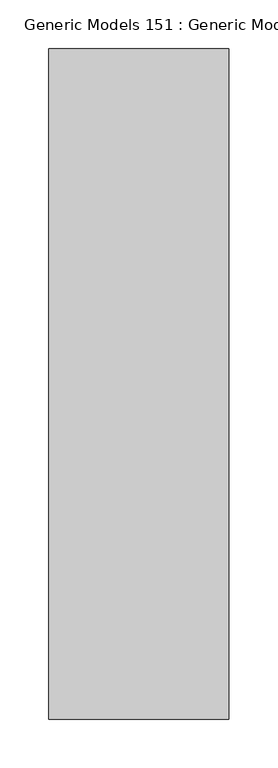
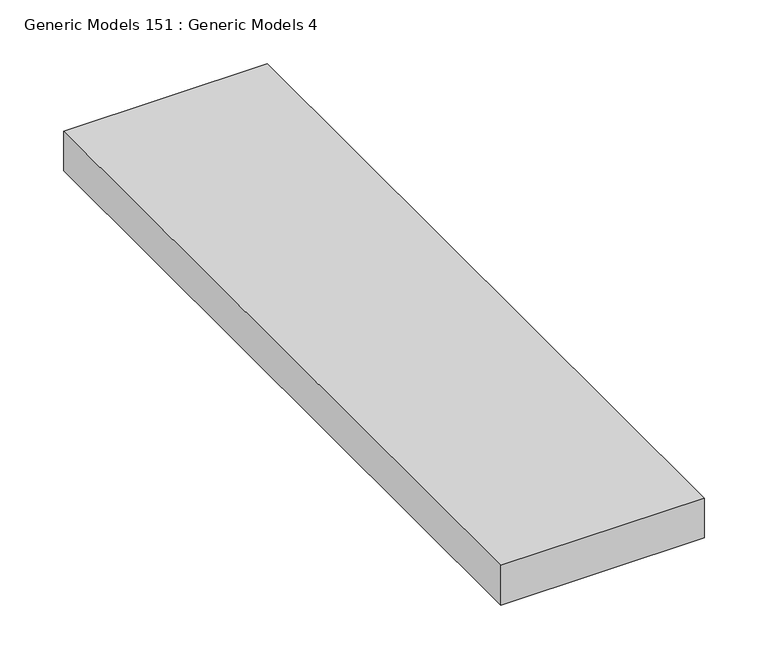
"""IFC4 building model written with IfcOpenShell, lengths in millimetres: proxy geometry, Generic Models 151 : Generic Models 4."""

import ifcopenshell
import ifcopenshell.guid

model = None  # the IFC model being written
_history = None  # IfcOwnerHistory: only IFC2X3 demands one
_inside = {}  # id of a spatial element -> (the spatial element, [elements in it])
_under = {}  # id of a project, library or spatial element -> (it, [spatial elements below it])
_declared = {}  # id of a project -> (the project, [libraries it declares])
_typed = {}  # id of a type object -> (the type object, [elements of that type])
_made_of = {}  # id of a material, layer set ... -> (it, [elements and type objects made of it])


def new_model(schema):
    """Start an empty IFC model of exactly this schema.

    Asked for "IFC4X3", IfcOpenShell would pick the latest addendum, in which some entities
    have other attributes; the version numbers below select the first issue.
    IFC2X3 requires an IfcOwnerHistory on every rooted entity: one is made here for all.
    """
    global model, _history
    if schema == "IFC4X3":
        model = ifcopenshell.file(schema_version=(4, 3, 0, 0))
    else:
        model = ifcopenshell.file(schema=schema)
    _inside.clear()
    _under.clear()
    _declared.clear()
    _typed.clear()
    _made_of.clear()
    _history = None
    if model.schema == "IFC2X3":
        org = make("IfcOrganization", Name="unknown")
        user = make(
            "IfcPersonAndOrganization",
            ThePerson=make("IfcPerson", FamilyName="unknown"),
            TheOrganization=org,
        )
        app = make(
            "IfcApplication",
            ApplicationDeveloper=org,
            Version="unknown",
            ApplicationFullName="unknown",
            ApplicationIdentifier="unknown",
        )
        _history = make(
            "IfcOwnerHistory",
            OwningUser=user,
            OwningApplication=app,
            ChangeAction="ADDED",
            CreationDate=0,
        )
    return model


def make(cls, **values):
    """One entity of the class cls with the attributes given. An attribute that is None is left unset."""
    return model.create_entity(
        cls, **{name: value for name, value in values.items() if value is not None}
    )


def rooted(cls, **values):
    """An entity with a GlobalId (a new one), such as an element, a storey or a relation."""
    return make(cls, GlobalId=ifcopenshell.guid.new(), OwnerHistory=_history, **values)


def si_unit(unit_type, name, prefix=None):
    """IfcSIUnit, for example si_unit("LENGTHUNIT", "METRE", prefix="MILLI")."""
    return make("IfcSIUnit", UnitType=unit_type, Prefix=prefix, Name=name)


def assignment(units):
    """IfcUnitAssignment: the units of a project."""
    return None if units is None else make("IfcUnitAssignment", Units=units)


def point(xyz):
    """IfcCartesianPoint."""
    return None if xyz is None else make("IfcCartesianPoint", Coordinates=xyz)


def direction(xyz):
    """IfcDirection."""
    return None if xyz is None else make("IfcDirection", DirectionRatios=xyz)


def frame(location, z_axis=None, x_axis=None):
    """IfcAxis2Placement3D, a coordinate frame: its origin and axes. An axis left out is left unset."""
    return make(
        "IfcAxis2Placement3D",
        Location=point(location),
        Axis=direction(z_axis),
        RefDirection=direction(x_axis),
    )


def origin():
    """The frame at (0, 0, 0) with its axes left unset."""
    return frame((0.0, 0.0, 0.0))


def place(relative_to, where):
    """IfcLocalPlacement: puts the frame where relative to a parent placement (None: the world)."""
    return make(
        "IfcLocalPlacement", PlacementRelTo=relative_to, RelativePlacement=where
    )


def context(
    kind, dimensions, precision=None, world=None, true_north=None, identifier=None
):
    """IfcGeometricRepresentationContext, for example the 3D "Model" context."""
    return make(
        "IfcGeometricRepresentationContext",
        ContextIdentifier=identifier,
        ContextType=kind,
        CoordinateSpaceDimension=dimensions,
        Precision=precision,
        WorldCoordinateSystem=world,
        TrueNorth=true_north,
    )


def project(units=None, contexts=None):
    """IfcProject with its units and contexts."""
    return rooted(
        "IfcProject",
        Name="project",
        RepresentationContexts=contexts,
        UnitsInContext=assignment(units),
    )


def spatial(cls, under=None, at=None, **own):
    """A site, building, storey or space (cls), placed at a placement, below another one or the project."""
    s = rooted(cls, ObjectPlacement=at, **own)
    if under is not None:
        _under.setdefault(under.id(), (under, []))[1].append(s)
    return s


def polyline(points):
    """IfcPolyline through the points."""
    return make("IfcPolyline", Points=[point(p) for p in points])


def outline(outer, holes=None, kind="AREA"):
    """IfcArbitraryClosedProfileDef: a profile drawn as a closed curve; with holes, ...WithVoids."""
    if holes is None:
        return make("IfcArbitraryClosedProfileDef", ProfileType=kind, OuterCurve=outer)
    return make(
        "IfcArbitraryProfileDefWithVoids",
        ProfileType=kind,
        OuterCurve=outer,
        InnerCurves=holes,
    )


def extrude(swept, where, along, depth):
    """IfcExtrudedAreaSolid: the profile swept, set in the frame where, extruded along a direction by depth."""
    return make(
        "IfcExtrudedAreaSolid",
        SweptArea=swept,
        Position=where,
        ExtrudedDirection=direction(along),
        Depth=depth,
    )


def shape(context_of_items, identifier, shape_type, items):
    """IfcShapeRepresentation: the items that make up one representation, for example the "Body"."""
    return make(
        "IfcShapeRepresentation",
        ContextOfItems=context_of_items,
        RepresentationIdentifier=identifier,
        RepresentationType=shape_type,
        Items=items,
    )


def source(mapping_origin, context_of_items, identifier, shape_type, items):
    """IfcRepresentationMap: a shape defined once, which mapped items show again and again."""
    return make(
        "IfcRepresentationMap",
        MappingOrigin=mapping_origin,
        MappedRepresentation=shape(context_of_items, identifier, shape_type, items),
    )


def transform(
    local_origin,
    x_axis=None,
    y_axis=None,
    z_axis=None,
    scale=None,
    scale2=None,
    scale3=None,
    uniform=True,
):
    """IfcCartesianTransformationOperator3D, or its non-uniform kind. x_axis, y_axis, z_axis: its Axis1, 2, 3."""
    if uniform:
        return make(
            "IfcCartesianTransformationOperator3D",
            Axis1=direction(x_axis),
            Axis2=direction(y_axis),
            LocalOrigin=point(local_origin),
            Scale=scale,
            Axis3=direction(z_axis),
        )
    return make(
        "IfcCartesianTransformationOperator3DnonUniform",
        Axis1=direction(x_axis),
        Axis2=direction(y_axis),
        LocalOrigin=point(local_origin),
        Scale=scale,
        Axis3=direction(z_axis),
        Scale2=scale2,
        Scale3=scale3,
    )


def mapped(mapping_source, mapping_target):
    """IfcMappedItem: shows the shape of a source again, moved by a transform."""
    return make(
        "IfcMappedItem", MappingSource=mapping_source, MappingTarget=mapping_target
    )


def made_of(thing, what):
    """Note that an element or type object is made of a material, layer set ...; save() writes the relation."""
    if what is not None:
        _made_of.setdefault(what.id(), (what, []))[1].append(thing)
    return thing


def element(
    cls,
    number,
    at=None,
    inside=None,
    cuts=None,
    type_object=None,
    material=None,
    context=None,
    identifier="Body",
    shape_type=None,
    held_by="IfcProductDefinitionShape",
    body=None,
    shapes=None,
    **own,
):
    """One element of the class cls, such as IfcWall. Its Tag is "e" and its number.

    at: its placement. inside: the storey or other place that contains it. cuts: it is an
    opening in that element (IfcRelVoidsElement). A single representation is given by context,
    identifier, shape_type and body (its items); several are given by shapes. held_by: the class
    of the entity that holds the representations. save() writes the other relations.
    """
    e = rooted(cls, Tag="e%d" % number, ObjectPlacement=at, **own)
    if body is not None:
        shapes = [shape(context, identifier, shape_type, body)]
    if shapes is not None:
        e.Representation = make(held_by, Representations=shapes)
    if inside is not None:
        _inside.setdefault(inside.id(), (inside, []))[1].append(e)
    if cuts is not None:
        rooted(
            "IfcRelVoidsElement", RelatingBuildingElement=cuts, RelatedOpeningElement=e
        )
    if type_object is not None:
        _typed.setdefault(type_object.id(), (type_object, []))[1].append(e)
    return made_of(e, material)


def aggregate(whole, parts):
    """IfcRelAggregates: a whole, such as a stair, and the parts it consists of."""
    return rooted("IfcRelAggregates", RelatingObject=whole, RelatedObjects=parts)


def save(model, path):
    """Write the relations noted so far, then the file.

    IfcRelAggregates (storeys below a building ...), IfcRelContainedInSpatialStructure (elements
    in a storey), IfcRelDefinesByType, IfcRelAssociatesMaterial and IfcRelDeclares: one each for
    every whole, place, type object, material and project.
    """
    for whole, parts in _under.values():
        aggregate(whole, parts)
    for where, things in _inside.values():
        rooted(
            "IfcRelContainedInSpatialStructure",
            RelatedElements=things,
            RelatingStructure=where,
        )
    for kind, things in _typed.values():
        rooted("IfcRelDefinesByType", RelatedObjects=things, RelatingType=kind)
    for what, things in _made_of.values():
        rooted("IfcRelAssociatesMaterial", RelatedObjects=things, RelatingMaterial=what)
    for by, libraries in _declared.values():
        rooted("IfcRelDeclares", RelatingContext=by, RelatedDefinitions=libraries)
    model.write(path)


def generic_models_151_generic_models_4_3b0b5e2b(model_context):
    return source(origin(), model_context, "Body", "SweptSolid", [
        extrude(outline(polyline([(-87.518833, 1085.2769662), (96.631167, 1085.2769662), (96.631167, 399.7309662), (-87.518833, 399.7309662), (-87.518833, 1085.2769662)])), frame((0.0, 0.0, 126518.4536306), z_axis=(0.0, 0.0, 1.0), x_axis=(1.0, 0.0, 0.0)), (0.0, 0.0, 1.0), 38.1),
    ])


if __name__ == "__main__":
    model = new_model("IFC4")
    model_context = context("Model", 3, world=origin())
    ifc_project = project(units=[si_unit("LENGTHUNIT", "METRE", prefix="MILLI")], contexts=[model_context])
    site = spatial("IfcSite", under=ifc_project)
    building = spatial("IfcBuilding", under=site)
    placement = place(None, origin())
    generic_models_151_generic_models_4_shape = generic_models_151_generic_models_4_3b0b5e2b(model_context)
    element("IfcBuildingElementProxy", 1, Name="Generic Models 151 : Generic Models 4", ObjectType="Generic Models 151 : Generic Models 4", at=placement, inside=building, context=model_context, shape_type="MappedRepresentation", body=[
        mapped(generic_models_151_generic_models_4_shape, transform((0.0, 0.0, 0.0), x_axis=(1.0, 0.0, 0.0), y_axis=(0.0, 1.0, 0.0), z_axis=(0.0, 0.0, 1.0))),
    ])
    save(model, "model.ifc")

# Revit data of these elements
# Element 1 (IfcBuildingElementProxy, "Generic Models 151 : Generic Models 4")
#   Materials on its faces: "_BLOCKING AS REQUIRED"
# Materials
#   "_BLOCKING AS REQUIRED": class "Generic", colour RGB 177 130 114, transparency 0, Cost = 0
